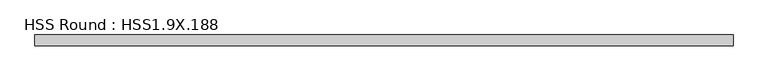
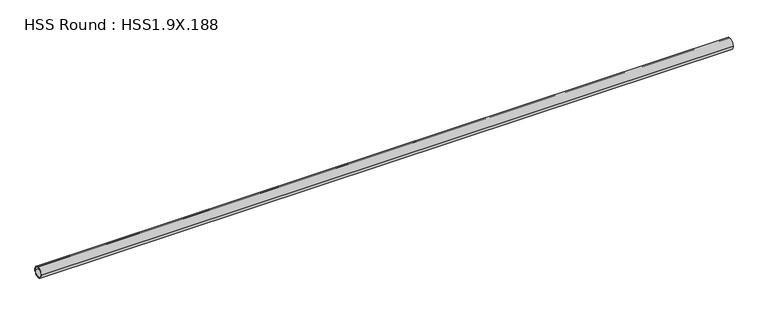
"""IFC4 building model written with IfcOpenShell, lengths in millimetres: member geometry, HSS Round : HSS1.9X.188."""

from ifc_helpers import new_model, si_unit, point, frame, origin, origin_2d, place, context, project, spatial, circle_curve, trimmed, segment, composite_curve, outline, extrude, source, transform, mapped, element, save


def hss_round_hss1_9x_188_f4985c19(model_context):
    return source(origin(), model_context, "Body", "SweptSolid", [
        extrude(outline(composite_curve([segment(trimmed(circle_curve(origin_2d(), 24.13), [point((-24.13, 0.0))], [point((24.13, 0.0))], False, "CARTESIAN"), True, "CONTINUOUS"), segment(trimmed(circle_curve(origin_2d(), 24.13), [point((24.13, 0.0))], [point((-24.13, 0.0))], False, "CARTESIAN"), True, "CONTINUOUS")], self_intersect=False), holes=[composite_curve([segment(trimmed(circle_curve(origin_2d(), 19.3548), [point((19.3548, 0.0))], [point((-19.3548, 0.0))], True, "CARTESIAN"), True, "CONTINUOUS"), segment(trimmed(circle_curve(origin_2d(), 19.3548), [point((-19.3548, 0.0))], [point((19.3548, 0.0))], True, "CARTESIAN"), True, "CONTINUOUS")], self_intersect=False)]), frame((-1560.9469018, 0.0, 0.0), z_axis=(1.0, 0.0, 0.0), x_axis=(0.0, 1.0, 0.0)), (0.0, 0.0, 1.0), 3050.6399702),
    ])


if __name__ == "__main__":
    model = new_model("IFC4")
    model_context = context("Model", 3, world=origin())
    ifc_project = project(units=[si_unit("LENGTHUNIT", "METRE", prefix="MILLI")], contexts=[model_context])
    site = spatial("IfcSite", under=ifc_project)
    building = spatial("IfcBuilding", under=site)
    placement = place(None, origin())
    hss_round_hss1_9x_188_shape = hss_round_hss1_9x_188_f4985c19(model_context)
    element("IfcMember", 1, ObjectType="HSS Round : HSS1.9X.188", at=placement, inside=building, context=model_context, shape_type="MappedRepresentation", body=[
        mapped(hss_round_hss1_9x_188_shape, transform((0.0, 0.0, 0.0), x_axis=(1.0, 0.0, 0.0), y_axis=(0.0, 1.0, 0.0), z_axis=(0.0, 0.0, 1.0))),
    ])
    save(model, "model.ifc")

# Revit data of these elements
# Type "HSS Round : HSS1.9X.188"
#   Section Name Key = "HSSRound 1.900x0.188"
#   Assembly Code = "B10"
#   Wall Nominal Thickness = 0.188"
#   Wall Design Thickness = 0.174"
#   Torsional Moment of Inertia = 0.71 in⁴
#   Torsional Modulus = 0.747 in³
#   Section Area = 0.943 in²
#   Plastic Modulus weak axis = 0.52 in³
#   Plastic Modulus strong axis = 0.52 in³
#   Nominal Weight = 3.44 lbf/ft
#   Moment of Inertia weak axis = 0.355 in⁴
#   Moment of Inertia strong axis = 0.355 in⁴
#   Elastic Modulus weak axis = 0.374 in³
#   Elastic Modulus strong axis = 0.374 in³
#   Diameter = 1.900"
#   Centroid Vertical = 0.950"
#   Centroid Horizontal = 0.950"
#   Length [instance default] = 5' - 0"
#   Structural Material [instance default] = Steel ASTM A500, Grade B, Round
#   Warping Constant = (empty or 0)
#   Principal Axes Angle = 0
# Element 1 (IfcMember, "HSS Round : HSS1.9X.188")
#   Structural Material = Steel ASTM A992
#   Materials on its faces: "Steel ASTM A992"
# Materials
#   "Steel ASTM A500, Grade B, Round": class "Metal", colour RGB 199 199 199, transparency 0, Description = "Carbon steel", Cost = 0
#   "Steel ASTM A992": class "Metal", colour RGB 199 199 199, transparency 0, Description = "Structural steel 50ksi", Cost = 0
